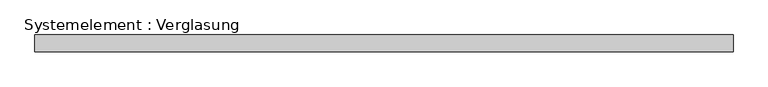
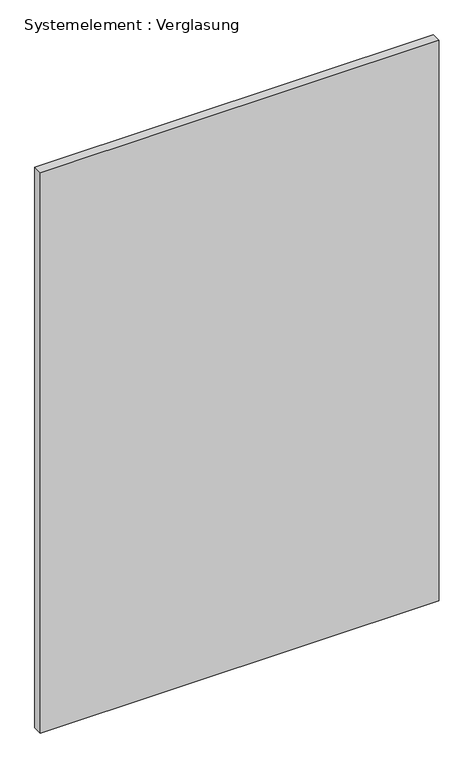
"""IFC4 building model written with IfcOpenShell, lengths in millimetres: plate geometry, Systemelement : Verglasung."""

import ifcopenshell
import ifcopenshell.guid

model = None  # the IFC model being written
_history = None  # IfcOwnerHistory: only IFC2X3 demands one
_inside = {}  # id of a spatial element -> (the spatial element, [elements in it])
_under = {}  # id of a project, library or spatial element -> (it, [spatial elements below it])
_declared = {}  # id of a project -> (the project, [libraries it declares])
_typed = {}  # id of a type object -> (the type object, [elements of that type])
_made_of = {}  # id of a material, layer set ... -> (it, [elements and type objects made of it])


def new_model(schema):
    """Start an empty IFC model of exactly this schema.

    Asked for "IFC4X3", IfcOpenShell would pick the latest addendum, in which some entities
    have other attributes; the version numbers below select the first issue.
    IFC2X3 requires an IfcOwnerHistory on every rooted entity: one is made here for all.
    """
    global model, _history
    if schema == "IFC4X3":
        model = ifcopenshell.file(schema_version=(4, 3, 0, 0))
    else:
        model = ifcopenshell.file(schema=schema)
    _inside.clear()
    _under.clear()
    _declared.clear()
    _typed.clear()
    _made_of.clear()
    _history = None
    if model.schema == "IFC2X3":
        org = make("IfcOrganization", Name="unknown")
        user = make(
            "IfcPersonAndOrganization",
            ThePerson=make("IfcPerson", FamilyName="unknown"),
            TheOrganization=org,
        )
        app = make(
            "IfcApplication",
            ApplicationDeveloper=org,
            Version="unknown",
            ApplicationFullName="unknown",
            ApplicationIdentifier="unknown",
        )
        _history = make(
            "IfcOwnerHistory",
            OwningUser=user,
            OwningApplication=app,
            ChangeAction="ADDED",
            CreationDate=0,
        )
    return model


def make(cls, **values):
    """One entity of the class cls with the attributes given. An attribute that is None is left unset."""
    return model.create_entity(
        cls, **{name: value for name, value in values.items() if value is not None}
    )


def rooted(cls, **values):
    """An entity with a GlobalId (a new one), such as an element, a storey or a relation."""
    return make(cls, GlobalId=ifcopenshell.guid.new(), OwnerHistory=_history, **values)


def si_unit(unit_type, name, prefix=None):
    """IfcSIUnit, for example si_unit("LENGTHUNIT", "METRE", prefix="MILLI")."""
    return make("IfcSIUnit", UnitType=unit_type, Prefix=prefix, Name=name)


def assignment(units):
    """IfcUnitAssignment: the units of a project."""
    return None if units is None else make("IfcUnitAssignment", Units=units)


def point(xyz):
    """IfcCartesianPoint."""
    return None if xyz is None else make("IfcCartesianPoint", Coordinates=xyz)


def direction(xyz):
    """IfcDirection."""
    return None if xyz is None else make("IfcDirection", DirectionRatios=xyz)


def frame(location, z_axis=None, x_axis=None):
    """IfcAxis2Placement3D, a coordinate frame: its origin and axes. An axis left out is left unset."""
    return make(
        "IfcAxis2Placement3D",
        Location=point(location),
        Axis=direction(z_axis),
        RefDirection=direction(x_axis),
    )


def origin():
    """The frame at (0, 0, 0) with its axes left unset."""
    return frame((0.0, 0.0, 0.0))


def origin_with_axes():
    """The frame at (0, 0, 0) with the z axis (0, 0, 1) and the x axis (1, 0, 0) written out."""
    return frame((0.0, 0.0, 0.0), z_axis=(0.0, 0.0, 1.0), x_axis=(1.0, 0.0, 0.0))


def place(relative_to, where):
    """IfcLocalPlacement: puts the frame where relative to a parent placement (None: the world)."""
    return make(
        "IfcLocalPlacement", PlacementRelTo=relative_to, RelativePlacement=where
    )


def context(
    kind, dimensions, precision=None, world=None, true_north=None, identifier=None
):
    """IfcGeometricRepresentationContext, for example the 3D "Model" context."""
    return make(
        "IfcGeometricRepresentationContext",
        ContextIdentifier=identifier,
        ContextType=kind,
        CoordinateSpaceDimension=dimensions,
        Precision=precision,
        WorldCoordinateSystem=world,
        TrueNorth=true_north,
    )


def project(units=None, contexts=None):
    """IfcProject with its units and contexts."""
    return rooted(
        "IfcProject",
        Name="project",
        RepresentationContexts=contexts,
        UnitsInContext=assignment(units),
    )


def spatial(cls, under=None, at=None, **own):
    """A site, building, storey or space (cls), placed at a placement, below another one or the project."""
    s = rooted(cls, ObjectPlacement=at, **own)
    if under is not None:
        _under.setdefault(under.id(), (under, []))[1].append(s)
    return s


def polyline(points):
    """IfcPolyline through the points."""
    return make("IfcPolyline", Points=[point(p) for p in points])


def outline(outer, holes=None, kind="AREA"):
    """IfcArbitraryClosedProfileDef: a profile drawn as a closed curve; with holes, ...WithVoids."""
    if holes is None:
        return make("IfcArbitraryClosedProfileDef", ProfileType=kind, OuterCurve=outer)
    return make(
        "IfcArbitraryProfileDefWithVoids",
        ProfileType=kind,
        OuterCurve=outer,
        InnerCurves=holes,
    )


def extrude(swept, where, along, depth):
    """IfcExtrudedAreaSolid: the profile swept, set in the frame where, extruded along a direction by depth."""
    return make(
        "IfcExtrudedAreaSolid",
        SweptArea=swept,
        Position=where,
        ExtrudedDirection=direction(along),
        Depth=depth,
    )


def shape(context_of_items, identifier, shape_type, items):
    """IfcShapeRepresentation: the items that make up one representation, for example the "Body"."""
    return make(
        "IfcShapeRepresentation",
        ContextOfItems=context_of_items,
        RepresentationIdentifier=identifier,
        RepresentationType=shape_type,
        Items=items,
    )


def source(mapping_origin, context_of_items, identifier, shape_type, items):
    """IfcRepresentationMap: a shape defined once, which mapped items show again and again."""
    return make(
        "IfcRepresentationMap",
        MappingOrigin=mapping_origin,
        MappedRepresentation=shape(context_of_items, identifier, shape_type, items),
    )


def transform(
    local_origin,
    x_axis=None,
    y_axis=None,
    z_axis=None,
    scale=None,
    scale2=None,
    scale3=None,
    uniform=True,
):
    """IfcCartesianTransformationOperator3D, or its non-uniform kind. x_axis, y_axis, z_axis: its Axis1, 2, 3."""
    if uniform:
        return make(
            "IfcCartesianTransformationOperator3D",
            Axis1=direction(x_axis),
            Axis2=direction(y_axis),
            LocalOrigin=point(local_origin),
            Scale=scale,
            Axis3=direction(z_axis),
        )
    return make(
        "IfcCartesianTransformationOperator3DnonUniform",
        Axis1=direction(x_axis),
        Axis2=direction(y_axis),
        LocalOrigin=point(local_origin),
        Scale=scale,
        Axis3=direction(z_axis),
        Scale2=scale2,
        Scale3=scale3,
    )


def mapped(mapping_source, mapping_target):
    """IfcMappedItem: shows the shape of a source again, moved by a transform."""
    return make(
        "IfcMappedItem", MappingSource=mapping_source, MappingTarget=mapping_target
    )


def made_of(thing, what):
    """Note that an element or type object is made of a material, layer set ...; save() writes the relation."""
    if what is not None:
        _made_of.setdefault(what.id(), (what, []))[1].append(thing)
    return thing


def element(
    cls,
    number,
    at=None,
    inside=None,
    cuts=None,
    type_object=None,
    material=None,
    context=None,
    identifier="Body",
    shape_type=None,
    held_by="IfcProductDefinitionShape",
    body=None,
    shapes=None,
    **own,
):
    """One element of the class cls, such as IfcWall. Its Tag is "e" and its number.

    at: its placement. inside: the storey or other place that contains it. cuts: it is an
    opening in that element (IfcRelVoidsElement). A single representation is given by context,
    identifier, shape_type and body (its items); several are given by shapes. held_by: the class
    of the entity that holds the representations. save() writes the other relations.
    """
    e = rooted(cls, Tag="e%d" % number, ObjectPlacement=at, **own)
    if body is not None:
        shapes = [shape(context, identifier, shape_type, body)]
    if shapes is not None:
        e.Representation = make(held_by, Representations=shapes)
    if inside is not None:
        _inside.setdefault(inside.id(), (inside, []))[1].append(e)
    if cuts is not None:
        rooted(
            "IfcRelVoidsElement", RelatingBuildingElement=cuts, RelatedOpeningElement=e
        )
    if type_object is not None:
        _typed.setdefault(type_object.id(), (type_object, []))[1].append(e)
    return made_of(e, material)


def aggregate(whole, parts):
    """IfcRelAggregates: a whole, such as a stair, and the parts it consists of."""
    return rooted("IfcRelAggregates", RelatingObject=whole, RelatedObjects=parts)


def save(model, path):
    """Write the relations noted so far, then the file.

    IfcRelAggregates (storeys below a building ...), IfcRelContainedInSpatialStructure (elements
    in a storey), IfcRelDefinesByType, IfcRelAssociatesMaterial and IfcRelDeclares: one each for
    every whole, place, type object, material and project.
    """
    for whole, parts in _under.values():
        aggregate(whole, parts)
    for where, things in _inside.values():
        rooted(
            "IfcRelContainedInSpatialStructure",
            RelatedElements=things,
            RelatingStructure=where,
        )
    for kind, things in _typed.values():
        rooted("IfcRelDefinesByType", RelatedObjects=things, RelatingType=kind)
    for what, things in _made_of.values():
        rooted("IfcRelAssociatesMaterial", RelatedObjects=things, RelatingMaterial=what)
    for by, libraries in _declared.values():
        rooted("IfcRelDeclares", RelatingContext=by, RelatedDefinitions=libraries)
    model.write(path)


def systemelement_verglasung_4c82009f(model_context):
    return source(origin(), model_context, "Body", "SweptSolid", [
        extrude(outline(polyline([(625.0000002, -15.0), (-625.0000002, -15.0), (-625.0000002, 15.0), (625.0000002, 15.0), (625.0000002, -15.0)])), origin_with_axes(), (0.0, 0.0, 1.0), 1856.6788019),
    ])


if __name__ == "__main__":
    model = new_model("IFC4")
    model_context = context("Model", 3, world=origin())
    ifc_project = project(units=[si_unit("LENGTHUNIT", "METRE", prefix="MILLI")], contexts=[model_context])
    site = spatial("IfcSite", under=ifc_project)
    building = spatial("IfcBuilding", under=site)
    placement = place(None, origin())
    systemelement_verglasung_shape = systemelement_verglasung_4c82009f(model_context)
    element("IfcPlate", 1, ObjectType="Systemelement : Verglasung", at=placement, inside=building, context=model_context, shape_type="MappedRepresentation", body=[
        mapped(systemelement_verglasung_shape, transform((0.0, 0.0, 0.0), x_axis=(1.0, 0.0, 0.0), y_axis=(0.0, 1.0, 0.0), z_axis=(0.0, 0.0, 1.0))),
    ])
    save(model, "model.ifc")

# Revit data of these elements
# Type "Systemelement : Verglasung"
#   Construction Type Id = "GSP4R"
#   Analytic Construction = "1/8 Zoll Pilkington-Verglasung einfach"
#   Visual Light Transmittance = 0.9
#   Solar Heat Gain Coefficient = 0.86
#   Heat Transfer Coefficient (U) = 6.7069 W/(m²·K)
# Element 1 (IfcPlate, "Systemelement : Verglasung")
#   Materials on its faces: "Glas"
# Materials
#   "Glas": class "Glas", colour RGB 0 0 255, transparency 0.75, Comments = "Render-Darstellung nicht aktualisiert ", Cost = 0
